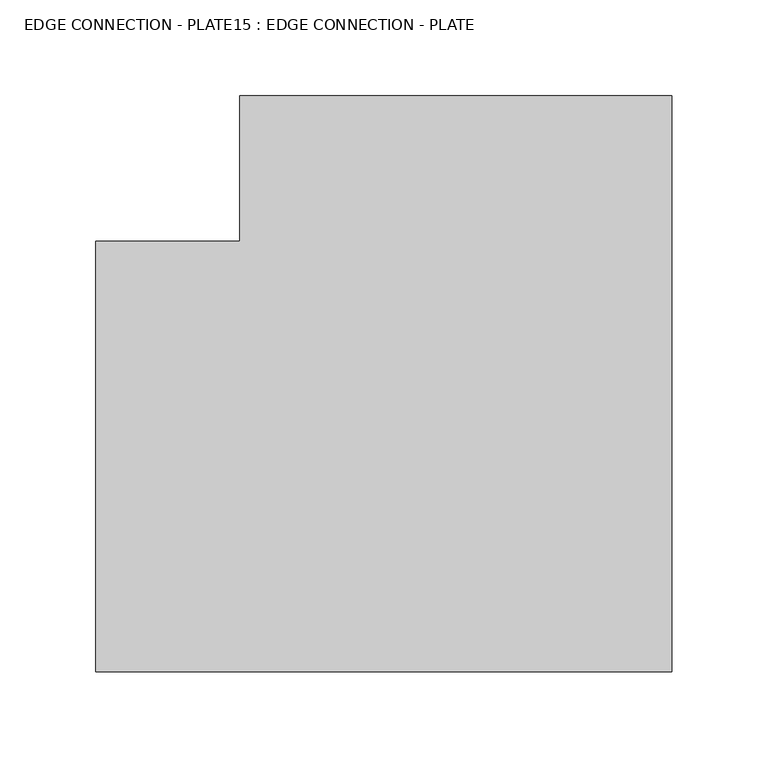
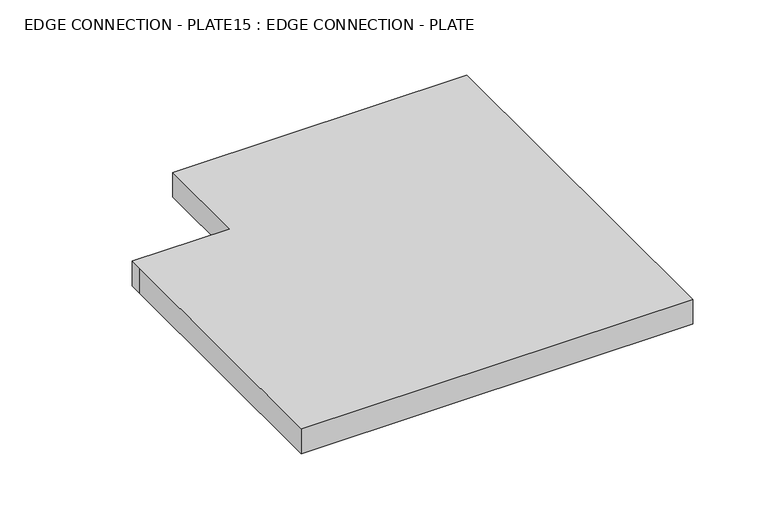
"""IFC4 building model written with IfcOpenShell, lengths in millimetres: fastener geometry, EDGE CONNECTION - PLATE15 : EDGE CONNECTION - PLATE."""

from ifc_helpers import new_model, si_unit, frame, origin, place, context, project, spatial, polyline, outline, extrude, source, transform, mapped, element, save


def edge_connection_plate15_edge_connection_plate_d07ce8ba(model_context):
    return source(origin(), model_context, "Body", "SweptSolid", [
        extrude(outline(polyline([(5700.0, 19499.5208589), (5700.0, 19713.9908589), (5700.0, 19723.9908589), (5774.862, 19723.9908589), (5774.862, 19799.5208589), (5784.862, 19799.5208589), (6000.0, 19799.5208589), (6000.0, 19499.5208589), (5700.0, 19499.5208589)])), frame((0.0, 0.0, 330.0), z_axis=(0.0, 0.0, 1.0), x_axis=(1.0, 0.0, 0.0)), (0.0, 0.0, 1.0), 20.0),
    ])


if __name__ == "__main__":
    model = new_model("IFC4")
    model_context = context("Model", 3, world=origin())
    ifc_project = project(units=[si_unit("LENGTHUNIT", "METRE", prefix="MILLI")], contexts=[model_context])
    site = spatial("IfcSite", under=ifc_project)
    building = spatial("IfcBuilding", under=site)
    placement = place(None, origin())
    edge_connection_plate15_edge_connection_plate_shape = edge_connection_plate15_edge_connection_plate_d07ce8ba(model_context)
    element("IfcFastener", 1, ObjectType="EDGE CONNECTION - PLATE15 : EDGE CONNECTION - PLATE", at=placement, inside=building, context=model_context, shape_type="MappedRepresentation", body=[
        mapped(edge_connection_plate15_edge_connection_plate_shape, transform((0.0, 0.0, 0.0), x_axis=(1.0, 0.0, 0.0), y_axis=(0.0, 1.0, 0.0), z_axis=(0.0, 0.0, 1.0))),
    ])
    save(model, "model.ifc")
